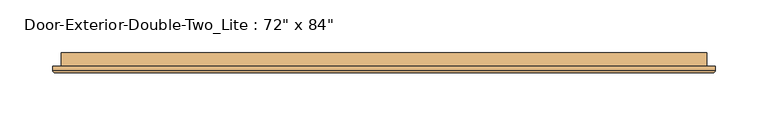
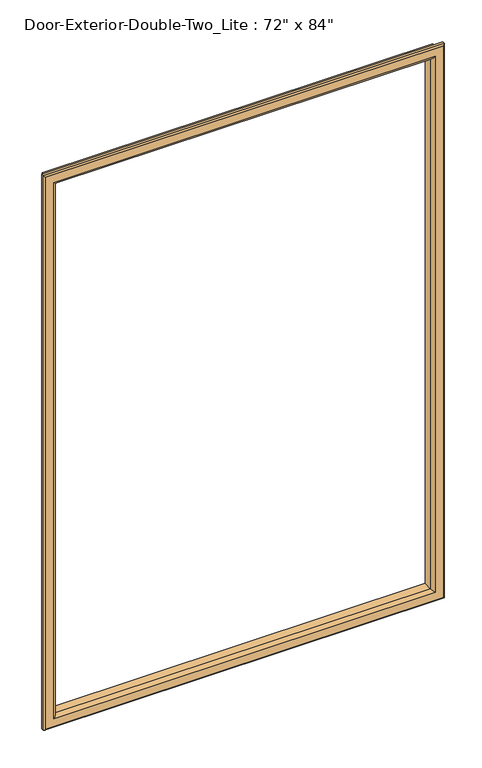
"""IFC4 building model written with IfcOpenShell, lengths in millimetres: door geometry."""

import ifcopenshell
import ifcopenshell.guid

model = None  # the IFC model being written
_history = None  # IfcOwnerHistory: only IFC2X3 demands one
_inside = {}  # id of a spatial element -> (the spatial element, [elements in it])
_under = {}  # id of a project, library or spatial element -> (it, [spatial elements below it])
_declared = {}  # id of a project -> (the project, [libraries it declares])
_typed = {}  # id of a type object -> (the type object, [elements of that type])
_made_of = {}  # id of a material, layer set ... -> (it, [elements and type objects made of it])


def new_model(schema):
    """Start an empty IFC model of exactly this schema.

    Asked for "IFC4X3", IfcOpenShell would pick the latest addendum, in which some entities
    have other attributes; the version numbers below select the first issue.
    IFC2X3 requires an IfcOwnerHistory on every rooted entity: one is made here for all.
    """
    global model, _history
    if schema == "IFC4X3":
        model = ifcopenshell.file(schema_version=(4, 3, 0, 0))
    else:
        model = ifcopenshell.file(schema=schema)
    _inside.clear()
    _under.clear()
    _declared.clear()
    _typed.clear()
    _made_of.clear()
    _history = None
    if model.schema == "IFC2X3":
        org = make("IfcOrganization", Name="unknown")
        user = make(
            "IfcPersonAndOrganization",
            ThePerson=make("IfcPerson", FamilyName="unknown"),
            TheOrganization=org,
        )
        app = make(
            "IfcApplication",
            ApplicationDeveloper=org,
            Version="unknown",
            ApplicationFullName="unknown",
            ApplicationIdentifier="unknown",
        )
        _history = make(
            "IfcOwnerHistory",
            OwningUser=user,
            OwningApplication=app,
            ChangeAction="ADDED",
            CreationDate=0,
        )
    return model


def make(cls, **values):
    """One entity of the class cls with the attributes given. An attribute that is None is left unset."""
    return model.create_entity(
        cls, **{name: value for name, value in values.items() if value is not None}
    )


def rooted(cls, **values):
    """An entity with a GlobalId (a new one), such as an element, a storey or a relation."""
    return make(cls, GlobalId=ifcopenshell.guid.new(), OwnerHistory=_history, **values)


def si_unit(unit_type, name, prefix=None):
    """IfcSIUnit, for example si_unit("LENGTHUNIT", "METRE", prefix="MILLI")."""
    return make("IfcSIUnit", UnitType=unit_type, Prefix=prefix, Name=name)


def assignment(units):
    """IfcUnitAssignment: the units of a project."""
    return None if units is None else make("IfcUnitAssignment", Units=units)


def point(xyz):
    """IfcCartesianPoint."""
    return None if xyz is None else make("IfcCartesianPoint", Coordinates=xyz)


def direction(xyz):
    """IfcDirection."""
    return None if xyz is None else make("IfcDirection", DirectionRatios=xyz)


def frame(location, z_axis=None, x_axis=None):
    """IfcAxis2Placement3D, a coordinate frame: its origin and axes. An axis left out is left unset."""
    return make(
        "IfcAxis2Placement3D",
        Location=point(location),
        Axis=direction(z_axis),
        RefDirection=direction(x_axis),
    )


def origin():
    """The frame at (0, 0, 0) with its axes left unset."""
    return frame((0.0, 0.0, 0.0))


def place(relative_to, where):
    """IfcLocalPlacement: puts the frame where relative to a parent placement (None: the world)."""
    return make(
        "IfcLocalPlacement", PlacementRelTo=relative_to, RelativePlacement=where
    )


def context(
    kind, dimensions, precision=None, world=None, true_north=None, identifier=None
):
    """IfcGeometricRepresentationContext, for example the 3D "Model" context."""
    return make(
        "IfcGeometricRepresentationContext",
        ContextIdentifier=identifier,
        ContextType=kind,
        CoordinateSpaceDimension=dimensions,
        Precision=precision,
        WorldCoordinateSystem=world,
        TrueNorth=true_north,
    )


def project(units=None, contexts=None):
    """IfcProject with its units and contexts."""
    return rooted(
        "IfcProject",
        Name="project",
        RepresentationContexts=contexts,
        UnitsInContext=assignment(units),
    )


def spatial(cls, under=None, at=None, **own):
    """A site, building, storey or space (cls), placed at a placement, below another one or the project."""
    s = rooted(cls, ObjectPlacement=at, **own)
    if under is not None:
        _under.setdefault(under.id(), (under, []))[1].append(s)
    return s


def ellipse_curve(where, semi_axis1, semi_axis2):
    """IfcEllipse in the frame where."""
    return make(
        "IfcEllipse", Position=where, SemiAxis1=semi_axis1, SemiAxis2=semi_axis2
    )


def shape(context_of_items, identifier, shape_type, items):
    """IfcShapeRepresentation: the items that make up one representation, for example the "Body"."""
    return make(
        "IfcShapeRepresentation",
        ContextOfItems=context_of_items,
        RepresentationIdentifier=identifier,
        RepresentationType=shape_type,
        Items=items,
    )


def source(mapping_origin, context_of_items, identifier, shape_type, items):
    """IfcRepresentationMap: a shape defined once, which mapped items show again and again."""
    return make(
        "IfcRepresentationMap",
        MappingOrigin=mapping_origin,
        MappedRepresentation=shape(context_of_items, identifier, shape_type, items),
    )


def transform(
    local_origin,
    x_axis=None,
    y_axis=None,
    z_axis=None,
    scale=None,
    scale2=None,
    scale3=None,
    uniform=True,
):
    """IfcCartesianTransformationOperator3D, or its non-uniform kind. x_axis, y_axis, z_axis: its Axis1, 2, 3."""
    if uniform:
        return make(
            "IfcCartesianTransformationOperator3D",
            Axis1=direction(x_axis),
            Axis2=direction(y_axis),
            LocalOrigin=point(local_origin),
            Scale=scale,
            Axis3=direction(z_axis),
        )
    return make(
        "IfcCartesianTransformationOperator3DnonUniform",
        Axis1=direction(x_axis),
        Axis2=direction(y_axis),
        LocalOrigin=point(local_origin),
        Scale=scale,
        Axis3=direction(z_axis),
        Scale2=scale2,
        Scale3=scale3,
    )


def mapped(mapping_source, mapping_target):
    """IfcMappedItem: shows the shape of a source again, moved by a transform."""
    return make(
        "IfcMappedItem", MappingSource=mapping_source, MappingTarget=mapping_target
    )


def made_of(thing, what):
    """Note that an element or type object is made of a material, layer set ...; save() writes the relation."""
    if what is not None:
        _made_of.setdefault(what.id(), (what, []))[1].append(thing)
    return thing


def element(
    cls,
    number,
    at=None,
    inside=None,
    cuts=None,
    type_object=None,
    material=None,
    context=None,
    identifier="Body",
    shape_type=None,
    held_by="IfcProductDefinitionShape",
    body=None,
    shapes=None,
    **own,
):
    """One element of the class cls, such as IfcWall. Its Tag is "e" and its number.

    at: its placement. inside: the storey or other place that contains it. cuts: it is an
    opening in that element (IfcRelVoidsElement). A single representation is given by context,
    identifier, shape_type and body (its items); several are given by shapes. held_by: the class
    of the entity that holds the representations. save() writes the other relations.
    """
    e = rooted(cls, Tag="e%d" % number, ObjectPlacement=at, **own)
    if body is not None:
        shapes = [shape(context, identifier, shape_type, body)]
    if shapes is not None:
        e.Representation = make(held_by, Representations=shapes)
    if inside is not None:
        _inside.setdefault(inside.id(), (inside, []))[1].append(e)
    if cuts is not None:
        rooted(
            "IfcRelVoidsElement", RelatingBuildingElement=cuts, RelatedOpeningElement=e
        )
    if type_object is not None:
        _typed.setdefault(type_object.id(), (type_object, []))[1].append(e)
    return made_of(e, material)


def aggregate(whole, parts):
    """IfcRelAggregates: a whole, such as a stair, and the parts it consists of."""
    return rooted("IfcRelAggregates", RelatingObject=whole, RelatedObjects=parts)


def save(model, path):
    """Write the relations noted so far, then the file.

    IfcRelAggregates (storeys below a building ...), IfcRelContainedInSpatialStructure (elements
    in a storey), IfcRelDefinesByType, IfcRelAssociatesMaterial and IfcRelDeclares: one each for
    every whole, place, type object, material and project.
    """
    for whole, parts in _under.values():
        aggregate(whole, parts)
    for where, things in _inside.values():
        rooted(
            "IfcRelContainedInSpatialStructure",
            RelatedElements=things,
            RelatingStructure=where,
        )
    for kind, things in _typed.values():
        rooted("IfcRelDefinesByType", RelatedObjects=things, RelatingType=kind)
    for what, things in _made_of.values():
        rooted("IfcRelAssociatesMaterial", RelatedObjects=things, RelatingMaterial=what)
    for by, libraries in _declared.values():
        rooted("IfcRelDeclares", RelatingContext=by, RelatedDefinitions=libraries)
    model.write(path)


def plane_surface(at):
    """IfcPlane: the flat surface through the origin of the frame at, square to its z axis."""
    return make("IfcPlane", Position=at)


def cylinder_surface(at, radius):
    """IfcCylindricalSurface: all points at the distance radius from the z axis of the frame at."""
    return make("IfcCylindricalSurface", Position=at, Radius=radius)


def advanced_brep(points, edges, surfaces, faces):
    """IfcAdvancedBrep: a solid bounded by faces that lie on surfaces and meet in shared edges.

    An edge is (start, end): straight between two places in points (the first is 0);
    or (start, end, curve); or (start, end, curve, False) where it runs against its curve.
    A face is (place in surfaces, loops), or (place, loops, False) where it looks against
    its surface's normal. A loop lists edges by number (the first is 1), with a minus sign
    where the edge is run from its end to its start. The first loop is the outer one.
    """
    corners = [point(p) for p in points]
    vertices = [make("IfcVertexPoint", VertexGeometry=c) for c in corners]
    made = []
    for start, end, *more in edges:
        made.append(
            make(
                "IfcEdgeCurve",
                EdgeStart=vertices[start],
                EdgeEnd=vertices[end],
                EdgeGeometry=more[0] if more else make("IfcPolyline", Points=[corners[start], corners[end]]),
                SameSense=more[1] if len(more) > 1 else True,
            )
        )
    hull = []
    for where, loops, *sense in faces:
        bounds = []
        for j, loop in enumerate(loops):
            ring = [make("IfcOrientedEdge", EdgeElement=made[abs(k) - 1], Orientation=k > 0) for k in loop]
            bounds.append(
                make(
                    "IfcFaceOuterBound" if j == 0 else "IfcFaceBound",
                    Bound=make("IfcEdgeLoop", EdgeList=ring),
                    Orientation=True,
                )
            )
        hull.append(make("IfcAdvancedFace", Bounds=bounds, FaceSurface=surfaces[where], SameSense=sense[0] if sense else True))
    return make("IfcAdvancedBrep", Outer=make("IfcClosedShell", CfsFaces=hull))


def door_d0d74375(model_context):
    return source(origin(), model_context, "Body", "AdvancedBrep", [
        advanced_brep(
        [(-762.0, 36.5125, 1117.6), (-762.0, 23.8125, 1117.6), (-762.0, 23.8125, 2016.125), (-762.0, 36.5125, 2016.125), (-750.0, 22.8125, 1129.6), (-750.0, 36.5125, 1129.6), (-750.0, 36.5125, 2004.125), (-750.0, 22.8125, 2004.125), (-755.0, 17.8125, 1124.6), (-755.0, 17.8125, 2009.125), (-770.0, 19.8125, 1109.6), (-768.0, 17.8125, 1111.6), (-768.0, 17.8125, 2022.125), (-770.0, 19.8125, 2024.125), (-770.0, 23.8125, 1109.6), (-770.0, 23.8125, 2024.125), (-152.4, 23.8125, 2016.125), (-152.4, 36.5125, 2016.125), (-164.4, 36.5125, 2004.125), (-164.4, 22.8125, 2004.125), (-159.4, 17.8125, 2009.125), (-146.4, 17.8125, 2022.125), (-144.4, 19.8125, 2024.125), (-144.4, 23.8125, 2024.125), (-152.4, 23.8125, 1117.6), (-152.4, 36.5125, 1117.6), (-164.4, 36.5125, 1129.6), (-164.4, 22.8125, 1129.6), (-159.4, 17.8125, 1124.6), (-146.4, 17.8125, 1111.6), (-144.4, 19.8125, 1109.6), (-144.4, 23.8125, 1109.6)],
        [
            (0, 1),
            (1, 2),
            (2, 3),
            (3, 0),
            (4, 5),
            (5, 6),
            (6, 7),
            (7, 4),
            (8, 4, ellipse_curve(frame((-755.0, 22.8125, 1124.6), z_axis=(-0.7071067811865475, 0.0, 0.7071067811865475), x_axis=(-0.7071067811865474, 0.0, -0.7071067811865476)), 7.0710678, 5.0)),
            (7, 9, ellipse_curve(frame((-755.0, 22.8125, 2009.125), z_axis=(-0.7071067811865475, 0.0, -0.7071067811865475), x_axis=(0.7071067811865474, 0.0, -0.7071067811865476)), 7.0710678, 5.0)),
            (9, 8),
            (10, 11, ellipse_curve(frame((-768.0, 19.8125, 1111.6), z_axis=(-0.7071067811865475, 0.0, 0.7071067811865475), x_axis=(-0.7071067811865474, 0.0, -0.7071067811865476)), 2.8284271, 2.0)),
            (11, 12),
            (12, 13, ellipse_curve(frame((-768.0, 19.8125, 2022.125), z_axis=(-0.7071067811865475, 0.0, -0.7071067811865475), x_axis=(0.7071067811865474, 0.0, -0.7071067811865476)), 2.8284271, 2.0)),
            (13, 10),
            (14, 10),
            (13, 15),
            (15, 14),
            (2, 16),
            (16, 17),
            (17, 3),
            (6, 18),
            (18, 19),
            (19, 7),
            (19, 20, ellipse_curve(frame((-159.4, 22.8125, 2009.125), z_axis=(-0.7071067811865475, 0.0, 0.7071067811865475), x_axis=(-0.7071067811865476, 0.0, -0.7071067811865474)), 7.0710678, 5.0)),
            (20, 9),
            (12, 21),
            (21, 22, ellipse_curve(frame((-146.4, 19.8125, 2022.125), z_axis=(-0.7071067811865475, 0.0, 0.7071067811865475), x_axis=(-0.7071067811865476, 0.0, -0.7071067811865474)), 2.8284271, 2.0)),
            (22, 13),
            (22, 23),
            (23, 15),
            (16, 24),
            (24, 25),
            (25, 17),
            (18, 26),
            (26, 27),
            (27, 19),
            (27, 28, ellipse_curve(frame((-159.4, 22.8125, 1124.6), z_axis=(0.7071067811865475, 0.0, 0.7071067811865475), x_axis=(-0.7071067811865474, 0.0, 0.7071067811865476)), 7.0710678, 5.0)),
            (28, 20),
            (21, 29),
            (29, 30, ellipse_curve(frame((-146.4, 19.8125, 1111.6), z_axis=(0.7071067811865475, 0.0, 0.7071067811865475), x_axis=(-0.7071067811865474, 0.0, 0.7071067811865476)), 2.8284271, 2.0)),
            (30, 22),
            (30, 31),
            (31, 23),
            (31, 14),
            (1, 24),
            (0, 25),
            (5, 26),
            (4, 27),
            (8, 28),
            (11, 29),
            (10, 30),
        ],
        [
            plane_surface(frame((-762.0, 23.8125, 1117.6), z_axis=(-1.0, 0.0, 0.0), x_axis=(0.0, 0.0, 1.0))),
            plane_surface(frame((-750.0, 36.5125, 1129.6), z_axis=(1.0, 0.0, 0.0), x_axis=(0.0, 0.0, 1.0))),
            cylinder_surface(frame((-755.0, 22.8125, 1117.6), z_axis=(0.0, 0.0, -1.0), x_axis=(-1.0, 0.0, 0.0)), 5.0),
            cylinder_surface(frame((-768.0, 19.8125, 1117.6), z_axis=(0.0, 0.0, -1.0), x_axis=(-1.0, 0.0, 0.0)), 2.0),
            plane_surface(frame((-770.0, 19.8125, 1109.6), z_axis=(-1.0, 0.0, 0.0), x_axis=(0.0, 0.0, 1.0))),
            plane_surface(frame((-762.0, 23.8125, 2016.125), z_axis=(0.0, 0.0, 1.0), x_axis=(1.0, 0.0, 0.0))),
            plane_surface(frame((-750.0, 36.5125, 2004.125), z_axis=(0.0, 0.0, -1.0), x_axis=(1.0, 0.0, 0.0))),
            cylinder_surface(frame((-762.0, 22.8125, 2009.125), z_axis=(-1.0, 0.0, 0.0), x_axis=(0.0, 0.0, 1.0)), 5.0),
            cylinder_surface(frame((-762.0, 19.8125, 2022.125), z_axis=(-1.0, 0.0, 0.0), x_axis=(0.0, 0.0, 1.0)), 2.0),
            plane_surface(frame((-770.0, 19.8125, 2024.125), z_axis=(0.0, 0.0, 1.0), x_axis=(1.0, 0.0, 0.0))),
            plane_surface(frame((-152.4, 23.8125, 2016.125), z_axis=(1.0, 0.0, 0.0), x_axis=(0.0, 0.0, -1.0))),
            plane_surface(frame((-164.4, 36.5125, 2004.125), z_axis=(-1.0, 0.0, 0.0), x_axis=(0.0, 0.0, -1.0))),
            cylinder_surface(frame((-159.4, 22.8125, 2016.125), z_axis=(0.0, 0.0, 1.0), x_axis=(1.0, 0.0, 0.0)), 5.0),
            cylinder_surface(frame((-146.4, 19.8125, 2016.125), z_axis=(0.0, 0.0, 1.0), x_axis=(1.0, 0.0, 0.0)), 2.0),
            plane_surface(frame((-144.4, 19.8125, 2024.125), z_axis=(1.0, 0.0, 0.0), x_axis=(0.0, 0.0, -1.0))),
            plane_surface(frame((-144.4, 23.8125, 1109.6), z_axis=(0.0, 1.0, 0.0), x_axis=(-1.0, 0.0, 0.0))),
            plane_surface(frame((-152.4, 23.8125, 1117.6), z_axis=(0.0, 0.0, -1.0), x_axis=(-1.0, 0.0, 0.0))),
            plane_surface(frame((-152.4, 36.5125, 1117.6), z_axis=(0.0, 1.0, 0.0), x_axis=(-1.0, 0.0, 0.0))),
            plane_surface(frame((-164.4, 36.5125, 1129.6), z_axis=(0.0, 0.0, 1.0), x_axis=(-1.0, 0.0, 0.0))),
            cylinder_surface(frame((-152.4, 22.8125, 1124.6), z_axis=(1.0, 0.0, 0.0), x_axis=(0.0, 0.0, -1.0)), 5.0),
            plane_surface(frame((-159.4, 17.8125, 1124.6), z_axis=(0.0, -1.0, 0.0), x_axis=(-1.0, 0.0, 0.0))),
            cylinder_surface(frame((-152.4, 19.8125, 1111.6), z_axis=(1.0, 0.0, 0.0), x_axis=(0.0, 0.0, -1.0)), 2.0),
            plane_surface(frame((-144.4, 19.8125, 1109.6), z_axis=(0.0, 0.0, -1.0), x_axis=(-1.0, 0.0, 0.0))),
        ],
        [
            (0, [[1, 2, 3, 4]]),
            (1, [[5, 6, 7, 8]]),
            (2, [[9, -8, 10, 11]]),
            (3, [[12, 13, 14, 15]]),
            (4, [[16, -15, 17, 18]]),
            (5, [[-3, 19, 20, 21]]),
            (6, [[-7, 22, 23, 24]]),
            (7, [[-10, -24, 25, 26]]),
            (8, [[-14, 27, 28, 29]]),
            (9, [[-17, -29, 30, 31]]),
            (10, [[-20, 32, 33, 34]]),
            (11, [[-23, 35, 36, 37]]),
            (12, [[-25, -37, 38, 39]]),
            (13, [[-28, 40, 41, 42]]),
            (14, [[-30, -42, 43, 44]]),
            (15, [[-31, -44, 45, -18], [46, -32, -19, -2]]),
            (16, [[-33, -46, -1, 47]]),
            (17, [[-21, -34, -47, -4], [48, -35, -22, -6]]),
            (18, [[-36, -48, -5, 49]]),
            (19, [[-38, -49, -9, 50]]),
            (20, [[51, -40, -27, -13], [-26, -39, -50, -11]]),
            (21, [[-41, -51, -12, 52]]),
            (22, [[-43, -52, -16, -45]]),
        ],
    ),
    ])


if __name__ == "__main__":
    model = new_model("IFC4")
    model_context = context("Model", 3, world=origin())
    ifc_project = project(units=[si_unit("LENGTHUNIT", "METRE", prefix="MILLI")], contexts=[model_context])
    site = spatial("IfcSite", under=ifc_project)
    building = spatial("IfcBuilding", under=site)
    placement = place(None, origin())
    door_shape = door_d0d74375(model_context)
    element("IfcDoor", 1, ObjectType="Door-Exterior-Double-Two_Lite : 72\" x 84\"", at=placement, inside=building, context=model_context, shape_type="MappedRepresentation", body=[
        mapped(door_shape, transform((0.0, 0.0, 0.0), x_axis=(1.0, 0.0, 0.0), y_axis=(0.0, 1.0, 0.0), z_axis=(0.0, 0.0, 1.0))),
    ])
    save(model, "model.ifc")

# Revit data of these elements
# Type "Door-Exterior-Double-Two_Lite : 72\" x 84\""
#   Type Mark = "20"
#   Assembly Code = "B2030100"
#   Analytic Construction = "Metal frame, double glass door"
#   Top Rail = 0' - 4 5/8"
#   Threshold Length [instance default] = 6' - 4"
#   Threshold Offset [instance default] = 0' - 0 1/2"
#   Thickness = 0' - 1 3/4"
#   Thermal Resistance (R) = 1.3794 (h·ft²·°F)/BTU
#   Swing Angle [instance default] = 90.00°
#   Strike Height = 3' - 4"
#   Stiles = 0' - 6"
#   SinglePanelWidth = 3' - 0"
#   Rough Width [instance default] = 6' - 4"
#   Rough Height [instance default] = 7' - 4"
#   MFOpeningHeight [instance default] = 0' - 4"
#   MFOpeningWidth [instance default] = 0' - 4"
#   Lock Rail = 0' - 8"
#   Inset Calculate [instance default] = 0' - 4"
#   Masonry Inset [instance default] = 0' - 1"
#   Height = 7' - 0"
#   Width = 6' - 0"
#   Heat Transfer Coefficient (U) = 0.7250 BTU/(h·ft²·°F)
#   Glass Thickness = 0' - 0 3/4"
#   Masonry Frame Depth = 0' - 5 3/4"
#   Bottom Rail = 0' - 10"
#   Threshold [instance default] = yes
#   Masonry Frame [instance default] = yes
#   Function = 1
#   Dry Wall Frame [instance default] = no
#   Threshold Material = none
#   Panic Bar Material = Metal - Stainless Steel
#   Panel Material = Metal - Painted - Grey
#   Glass Stop Material = Metal - Painted - Grey
#   Frame Material = Metal - Painted - Grey
#   Exterior Pull Material = Metal - Stainless Steel
#   Visual Light Transmittance = 0
#   Solar Heat Gain Coefficient = 0
#   Wall Closure = (empty or 0)
# Element 1 (IfcDoor, "Door-Exterior-Double-Two_Lite : 72\" x 84\"")
#   Threshold Length = 6' - 0"
#   Rough Width = 6' - 2 1/2"
#   Rough Height = 7' - 1 1/4"
#   MFOpeningHeight = 0' - 1 1/4"
#   MFOpeningWidth = 0' - 2 1/2"
#   Inset Calculate = 0' - 3"
#   Masonry Frame = no
#   Dry Wall Frame = yes
#   Materials on its faces: "Metal - Painted - Grey", "Metal - Stainless Steel", "Glass"
# Materials
#   "Metal - Stainless Steel": class "Metal", colour RGB 247 247 247, transparency 0
#   "Metal - Painted - Grey": class "Paint", colour RGB 104 104 104, transparency 0, Cost = 0
#   "Glass": class "Glass", colour RGB 0 128 192, transparency 0.75, Description = "Soda Lime Glass", Cost = 0
